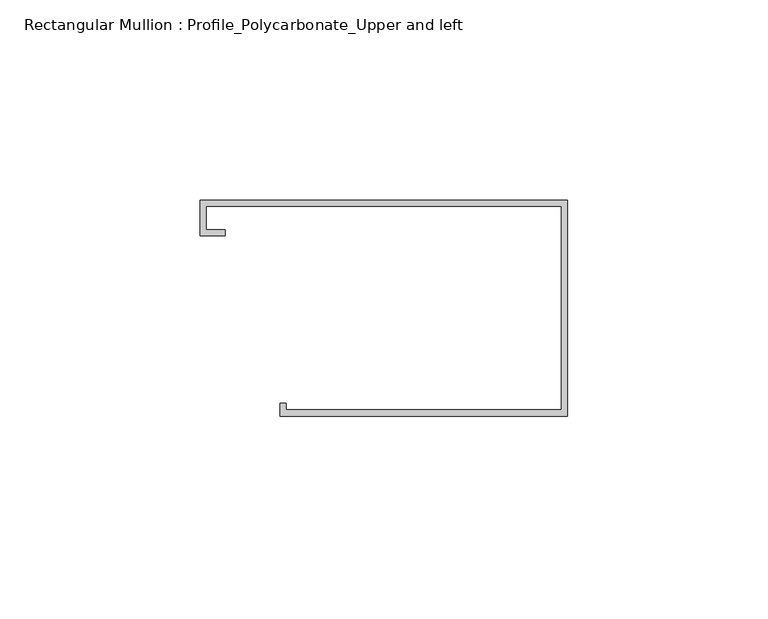
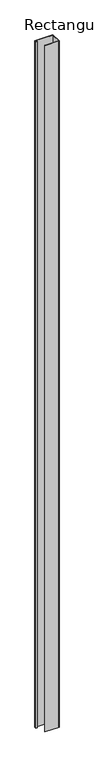
"""IFC4 building model written with IfcOpenShell, lengths in millimetres: member geometry, Rectangular Mullion : Profile_Polycarbonate_Upper and left."""

from ifc_helpers import new_model, si_unit, frame, origin, place, context, project, spatial, polyline, outline, extrude, source, transform, mapped, element, save


def rectangular_mullion_profile_polycarbonate_upper_and_left_7b20e4a8(model_context):
    return source(origin(), model_context, "Body", "SweptSolid", [
        extrude(outline(polyline([(0.0, 28.984575), (0.0, -25.015825), (-71.9836, -25.015825), (-71.9836, -21.840825), (-70.3961, -21.840825), (-70.3961, -23.428325), (-1.5875, -23.428325), (-1.5875, 27.397075), (-90.4113, 27.397075), (-90.4113, 21.580475), (-85.6488, 21.580475), (-85.6488, 19.992975), (-91.9988, 19.992975), (-91.9988, 28.984575), (0.0, 28.984575)])), frame((0.0, 0.0, -3697.323634), z_axis=(0.0, 0.0, 1.0), x_axis=(1.0, 0.0, 0.0)), (0.0, 0.0, 1.0), 3697.323634),
    ])


if __name__ == "__main__":
    model = new_model("IFC4")
    model_context = context("Model", 3, world=origin())
    ifc_project = project(units=[si_unit("LENGTHUNIT", "METRE", prefix="MILLI")], contexts=[model_context])
    site = spatial("IfcSite", under=ifc_project)
    building = spatial("IfcBuilding", under=site)
    placement = place(None, origin())
    rectangular_mullion_profile_polycarbonate_upper_and_left_shape = rectangular_mullion_profile_polycarbonate_upper_and_left_7b20e4a8(model_context)
    element("IfcMember", 1, ObjectType="Rectangular Mullion : Profile_Polycarbonate_Upper and left", at=placement, inside=building, context=model_context, shape_type="MappedRepresentation", body=[
        mapped(rectangular_mullion_profile_polycarbonate_upper_and_left_shape, transform((0.0, 0.0, 0.0), x_axis=(1.0, 0.0, 0.0), y_axis=(0.0, 1.0, 0.0), z_axis=(0.0, 0.0, 1.0))),
    ])
    save(model, "model.ifc")

# Revit data of these elements
# Type "Rectangular Mullion : Profile_Polycarbonate_Upper and left"
#   built-in parameter 1007322 = 0.177167 (stored number, unit not read)
#   built-in parameter 1007321 = 0.00520833 (stored number, unit not read)
#   built-in parameter 1007320 = 0 (stored number, unit not read)
